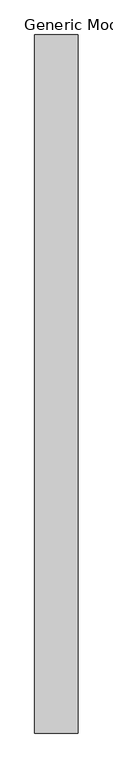
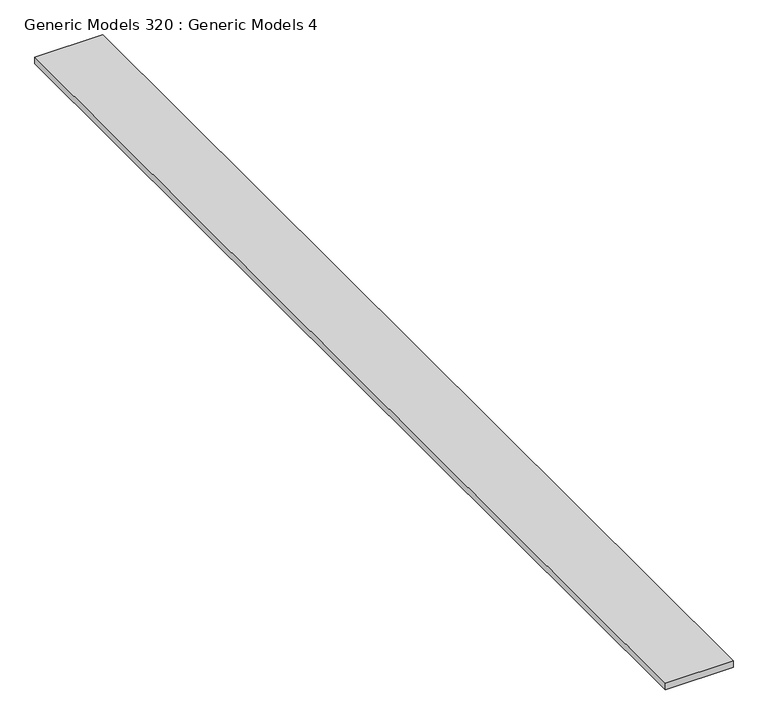
"""IFC4 building model written with IfcOpenShell, lengths in millimetres: proxy geometry, Generic Models 320 : Generic Models 4."""

from ifc_helpers import new_model, si_unit, frame, origin, place, context, project, spatial, polyline, outline, extrude, source, transform, mapped, element, save


def generic_models_320_generic_models_4_d83547cd(model_context):
    return source(origin(), model_context, "Body", "SweptSolid", [
        extrude(outline(polyline([(-5937.4236296, -5493.3230338), (-6426.3736296, -5493.3230338), (-6426.3736296, 2393.3769662), (-5937.4236296, 2393.3769662), (-5937.4236296, -5493.3230338)])), frame((0.0, 0.0, 123005.596), z_axis=(0.0, 0.0, 1.0), x_axis=(1.0, 0.0, 0.0)), (0.0, 0.0, 1.0), 50.8),
    ])


if __name__ == "__main__":
    model = new_model("IFC4")
    model_context = context("Model", 3, world=origin())
    ifc_project = project(units=[si_unit("LENGTHUNIT", "METRE", prefix="MILLI")], contexts=[model_context])
    site = spatial("IfcSite", under=ifc_project)
    building = spatial("IfcBuilding", under=site)
    placement = place(None, origin())
    generic_models_320_generic_models_4_shape = generic_models_320_generic_models_4_d83547cd(model_context)
    element("IfcBuildingElementProxy", 1, Name="Generic Models 320 : Generic Models 4", ObjectType="Generic Models 320 : Generic Models 4", at=placement, inside=building, context=model_context, shape_type="MappedRepresentation", body=[
        mapped(generic_models_320_generic_models_4_shape, transform((0.0, 0.0, 0.0), x_axis=(1.0, 0.0, 0.0), y_axis=(0.0, 1.0, 0.0), z_axis=(0.0, 0.0, 1.0))),
    ])
    save(model, "model.ifc")

# Revit data of these elements
# Element 1 (IfcBuildingElementProxy, "Generic Models 320 : Generic Models 4")
#   Materials on its faces: "_2\" SAND"
# Materials
#   "_2\" SAND": class "Generic", colour RGB 245 226 173, transparency 0, Cost = 0
